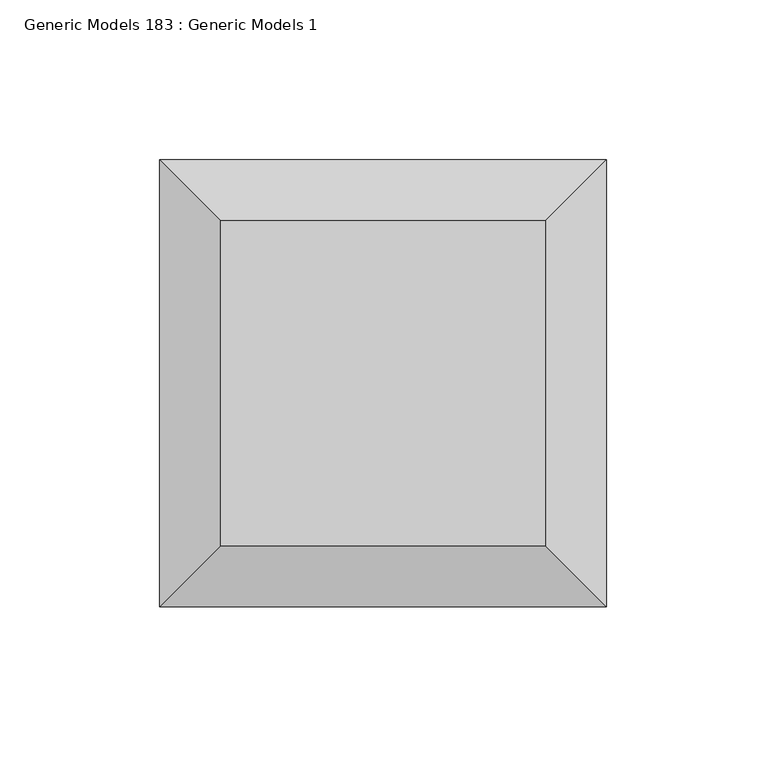
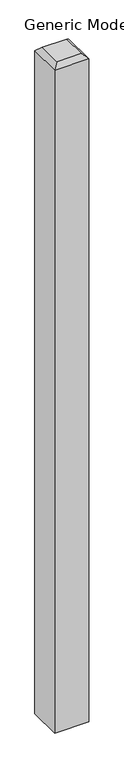
"""IFC4 building model written with IfcOpenShell, lengths in millimetres: proxy geometry, Generic Models 183 : Generic Models 1."""

from ifc_helpers import new_model, si_unit, origin, place, context, project, spatial, faceted_brep, source, transform, mapped, element, save


def generic_models_183_generic_models_1_4255d89c(model_context):
    return source(origin(), model_context, "Body", "Brep", [
        faceted_brep([(54227.4125, 528.6375, -1066.8), (54087.7125, 528.6375, -1066.8), (54087.7125, 528.6375, 1809.75), (54227.4125, 528.6375, 1809.75), (54227.4125, 388.9375, -1066.8), (54227.4125, 388.9375, 1809.75), (54087.7125, 388.9375, 1809.75), (54087.7125, 388.9375, -1066.8), (54106.7625, 407.9875, 1828.8), (54208.3625, 407.9875, 1828.8), (54208.3625, 509.5875, 1828.8), (54106.7625, 509.5875, 1828.8)], [[[0, 1, 2, 3]], [[4, 5, 6, 7]], [[1, 0, 4, 7]], [[2, 1, 7, 6]], [[8, 9, 10, 11]], [[0, 3, 5, 4]], [[2, 6, 8, 11]], [[5, 3, 10, 9]], [[6, 5, 9, 8]], [[3, 2, 11, 10]]]),
    ])


if __name__ == "__main__":
    model = new_model("IFC4")
    model_context = context("Model", 3, world=origin())
    ifc_project = project(units=[si_unit("LENGTHUNIT", "METRE", prefix="MILLI")], contexts=[model_context])
    site = spatial("IfcSite", under=ifc_project)
    building = spatial("IfcBuilding", under=site)
    placement = place(None, origin())
    generic_models_183_generic_models_1_shape = generic_models_183_generic_models_1_4255d89c(model_context)
    element("IfcBuildingElementProxy", 1, Name="Generic Models 183 : Generic Models 1", ObjectType="Generic Models 183 : Generic Models 1", at=placement, inside=building, context=model_context, shape_type="MappedRepresentation", body=[
        mapped(generic_models_183_generic_models_1_shape, transform((0.0, 0.0, 0.0), x_axis=(1.0, 0.0, 0.0), y_axis=(0.0, 1.0, 0.0), z_axis=(0.0, 0.0, 1.0))),
    ])
    save(model, "model.ifc")

# Revit data of these elements
# Element 1 (IfcBuildingElementProxy, "Generic Models 183 : Generic Models 1")
#   Materials on its faces: "TREATED 6X6 POST"
# Materials
#   "TREATED 6X6 POST": class "Wood", colour RGB 234 198 147, transparency 0, Description = "Pinus Echinata", Cost = 0
